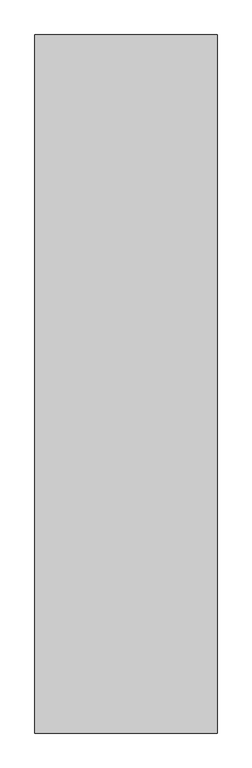
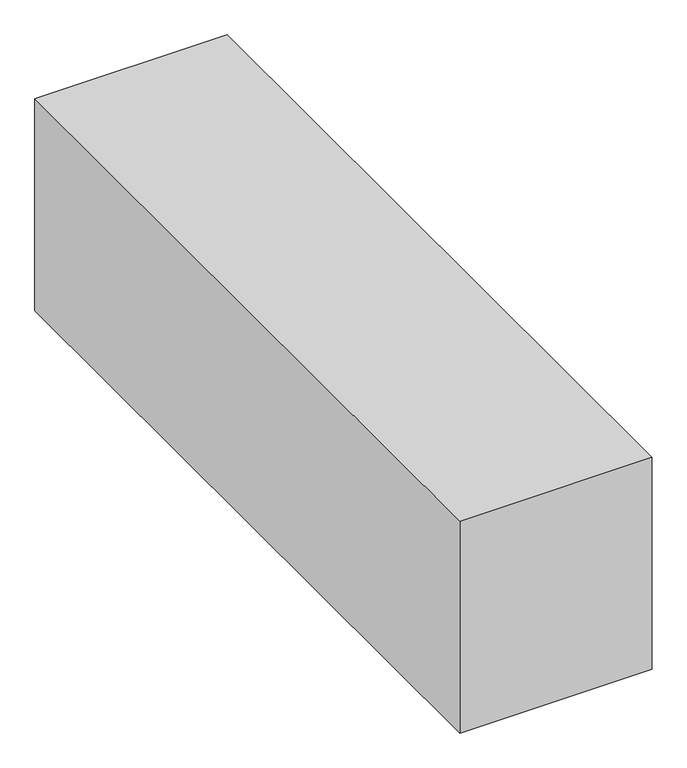
"""IFC4 building model written with IfcOpenShell, lengths in millimetres: proxy geometry, Space Planning Box_hec : Space Planning Box_hec."""

from ifc_helpers import new_model, si_unit, origin, origin_with_axes, place, context, project, spatial, polyline, outline, extrude, source, transform, mapped, element, save


def generic_models_f1f4091a(model_context):
    return source(origin(), model_context, "Body", "SweptSolid", [
        extrude(outline(polyline([(1500.0, 5750.0), (1500.0, -5750.0), (-1500.0, -5750.0), (-1500.0, 5750.0), (1500.0, 5750.0)])), origin_with_axes(), (0.0, 0.0, 1.0), 3500.0),
    ])


if __name__ == "__main__":
    model = new_model("IFC4")
    model_context = context("Model", 3, world=origin())
    ifc_project = project(units=[si_unit("LENGTHUNIT", "METRE", prefix="MILLI")], contexts=[model_context])
    site = spatial("IfcSite", under=ifc_project)
    building = spatial("IfcBuilding", under=site)
    placement = place(None, origin())
    generic_models_shape = generic_models_f1f4091a(model_context)
    element("IfcBuildingElementProxy", 1, Name="Space Planning Box_hec : Space Planning Box_hec", ObjectType="Space Planning Box_hec : Space Planning Box_hec", at=placement, inside=building, context=model_context, shape_type="MappedRepresentation", body=[
        mapped(generic_models_shape, transform((0.0, 0.0, 0.0), x_axis=(1.0, 0.0, 0.0), y_axis=(0.0, 1.0, 0.0), z_axis=(0.0, 0.0, 1.0))),
    ])
    save(model, "model.ifc")

# Revit data of these elements
# Type "Space Planning Box_hec : Space Planning Box_hec"
#   Type Comments = "..."
#   Room Name [instance default] = "?"
#   Interior Finish [instance default] = ""
#   Exterior Finish [instance default] = ""
#   Department [instance default] = ""
#   Assembly Code = "..."
#   ceiling height [instance default] = 0
#   Width [instance default] = 1524 mm
#   Program Area [instance default] = 0.00 m²
#   Length [instance default] = 1524 mm
#   Height [instance default] = 1524 mm
#   Area [instance default] = 2.32258 m²
#   Fill Color [instance default] = Cyan
#   Default Elevation = 0
# Element 1 (IfcBuildingElementProxy, "Space Planning Box_hec : Space Planning Box_hec")
#   Room Name = "Document Room"
#   Exterior Finish = "RF1..N/A,,N/A..N/A..N/A"
#   Department = "AR"
#   Width = 3000 mm
#   Program Area = 34.50 m²
#   Length = 11500 mm
#   Height = 3500 mm
#   Area = 34.50 m²
#   Materials on its faces: "Cyan"
# Materials
#   "Cyan": class "Generic", colour RGB 0 255 255, transparency 0.2, Cost = 0
